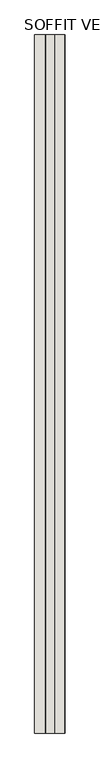
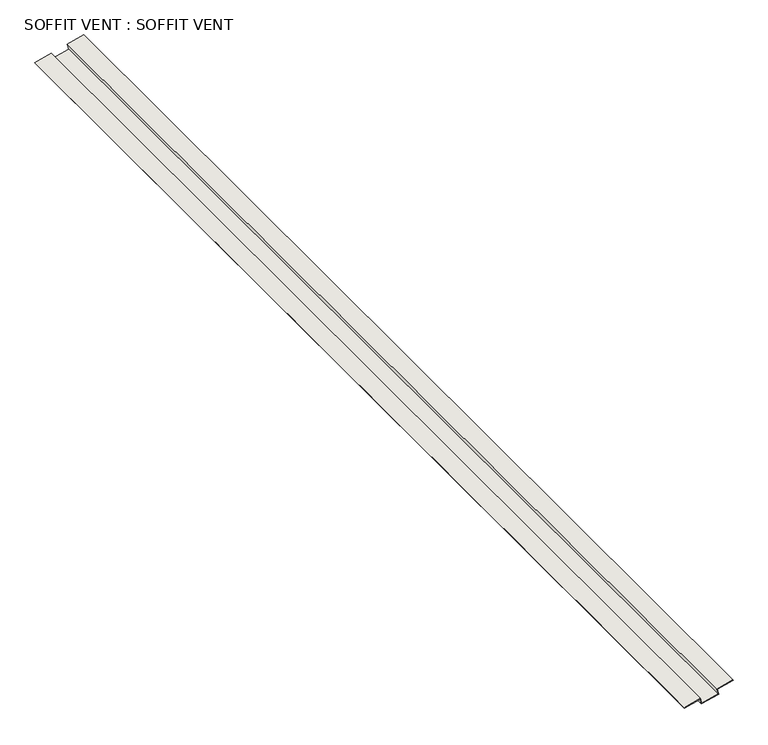
"""IFC4 building model written with IfcOpenShell, lengths in millimetres: wall geometry, SOFFIT VENT : SOFFIT VENT."""

from ifc_helpers import new_model, si_unit, frame, origin, place, context, project, spatial, polyline, outline, extrude, source, transform, mapped, element, save


def soffit_vent_soffit_vent_20fbd443(model_context):
    return source(origin(), model_context, "Body", "SweptSolid", [
        extrude(outline(polyline([(2354.1160886, 17868.9059296), (2337.1749752, 17873.1412079), (2324.8541655, 17823.8579689), (2341.7952789, 17819.6226906), (2329.4744691, 17770.3394516), (2327.9343679, 17770.7244769), (2339.8701524, 17818.4676147), (2322.929039, 17822.702893), (2336.0198993, 17875.0663345), (2352.9610127, 17870.8310561), (2364.8967972, 17918.5741939), (2366.4368984, 17918.1891686), (2354.1160886, 17868.9059296)])), frame((0.0, -3415.0384634, 0.0), z_axis=(0.0, 1.0, 0.0), x_axis=(0.0, 0.0, 1.0)), (0.0, 0.0, 1.0), 3403.6),
    ])


if __name__ == "__main__":
    model = new_model("IFC4")
    model_context = context("Model", 3, world=origin())
    ifc_project = project(units=[si_unit("LENGTHUNIT", "METRE", prefix="MILLI")], contexts=[model_context])
    site = spatial("IfcSite", under=ifc_project)
    building = spatial("IfcBuilding", under=site)
    placement = place(None, origin())
    soffit_vent_soffit_vent_shape = soffit_vent_soffit_vent_20fbd443(model_context)
    element("IfcWall", 1, ObjectType="SOFFIT VENT : SOFFIT VENT", at=placement, inside=building, context=model_context, shape_type="MappedRepresentation", body=[
        mapped(soffit_vent_soffit_vent_shape, transform((0.0, 0.0, 0.0), x_axis=(1.0, 0.0, 0.0), y_axis=(0.0, 1.0, 0.0), z_axis=(0.0, 0.0, 1.0))),
    ])
    save(model, "model.ifc")

# Revit data of these elements
# Element 1 (IfcWall, "SOFFIT VENT : SOFFIT VENT")
#   Materials on its faces: "LINEAR SOFFIT VENT"
# Materials
#   "LINEAR SOFFIT VENT": class "Metal", colour RGB 247 247 247, transparency 0, Description = "Aluminum 6061", Cost = 0
